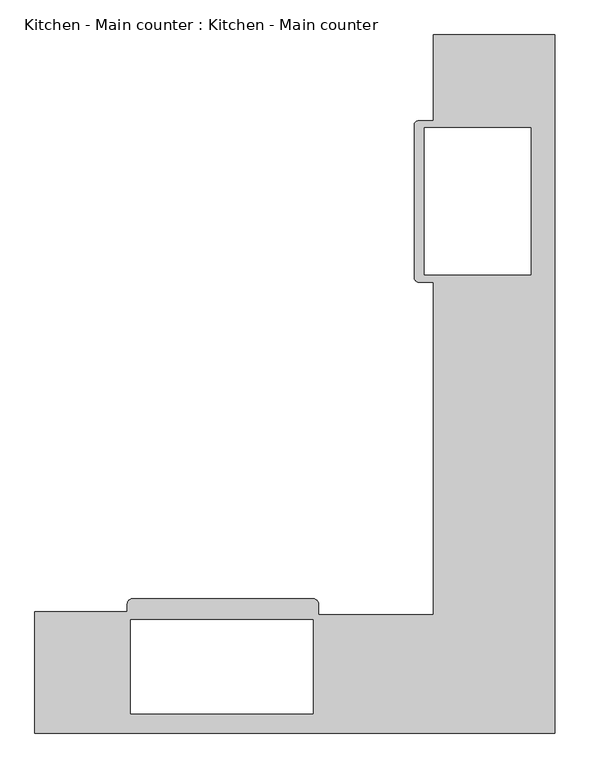
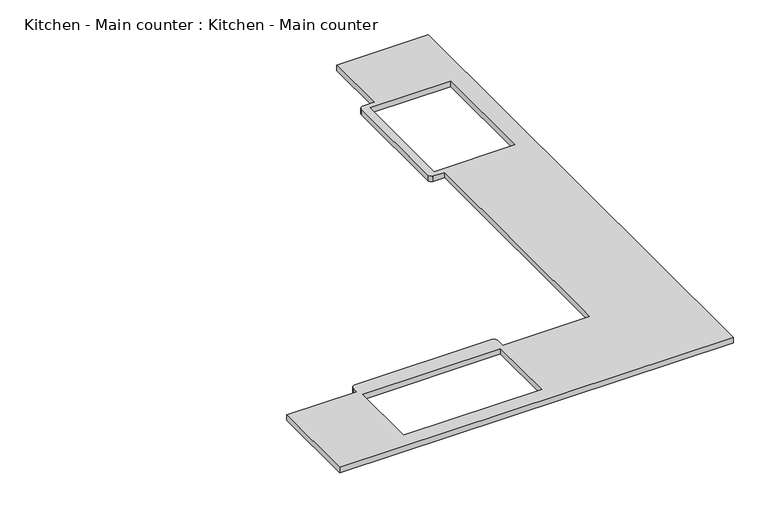
"""IFC4 building model written with IfcOpenShell, lengths in millimetres: furniture geometry, Kitchen - Main counter : Kitchen - Main counter."""

from ifc_helpers import new_model, si_unit, point, frame, frame_2d, origin, place, context, project, spatial, polyline, circle_curve, trimmed, segment, composite_curve, outline, extrude, source, transform, mapped, element, save


def kitchen_main_counter_kitchen_main_counter_9cb608c1(model_context):
    return source(origin(), model_context, "Body", "SweptSolid", [
        extrude(outline(composite_curve([segment(polyline([(5731.3758497, 9294.8125), (6195.1480033, 9294.8125), (6195.1480033, 9332.9125)]), True, "CONTINUOUS"), segment(trimmed(circle_curve(frame_2d((6220.5480033, 9332.9125)), 25.4), [point((6195.1480033, 9332.9125))], [point((6220.5480033, 9358.3125))], False, "CARTESIAN"), True, "CONTINUOUS"), segment(polyline([(6220.5480033, 9358.3125), (7128.4113603, 9358.3125)]), True, "CONTINUOUS"), segment(trimmed(circle_curve(frame_2d((7128.4113603, 9332.9125)), 25.4), [point((7128.4113603, 9358.3125))], [point((7153.8113603, 9332.9125))], False, "CARTESIAN"), True, "CONTINUOUS"), segment(polyline([(7153.8113603, 9332.9125), (7153.8113603, 9278.0953401), (7731.8480033, 9278.0953401), (7731.8480033, 10945.5241338), (7654.0605033, 10945.5241338)]), True, "CONTINUOUS"), segment(trimmed(circle_curve(frame_2d((7661.4688367, 10970.9241338)), 26.4583333), [point((7654.0605033, 10945.5241338))], [point((7635.0105033, 10970.9241338))], False, "CARTESIAN"), True, "CONTINUOUS"), segment(polyline([(7635.0105033, 10970.9241338), (7635.0105033, 11732.9241338)]), True, "CONTINUOUS"), segment(trimmed(circle_curve(frame_2d((7657.4611436, 11732.9241338)), 22.4506403), [point((7635.0105033, 11732.9241338))], [point((7657.4611436, 11755.3747741))], False, "CARTESIAN"), True, "CONTINUOUS"), segment(polyline([(7657.4611436, 11755.3747741), (7731.8480033, 11755.3747741), (7731.8480033, 12185.65), (8339.8605033, 12185.65), (8339.8605033, 8685.2125), (5731.3758497, 8685.2125), (5731.3758497, 9294.8125)]), True, "CONTINUOUS")], self_intersect=False), holes=[polyline([(7685.8105033, 10983.6241338), (8219.2105033, 10983.6241338), (8219.2105033, 11720.2241338), (7685.8105033, 11720.2241338), (7685.8105033, 11351.9241338), (7685.8105033, 10983.6241338)]), polyline([(7126.2875, 9254.5007015), (6211.8875, 9254.5007015), (6211.8875, 8783.3960572), (7126.2875, 8783.3960572), (7126.2875, 9254.5007015)])]), frame((0.0, 0.0, 876.3), z_axis=(0.0, 0.0, 1.0), x_axis=(1.0, 0.0, 0.0)), (0.0, 0.0, 1.0), 38.0405752),
    ])


if __name__ == "__main__":
    model = new_model("IFC4")
    model_context = context("Model", 3, world=origin())
    ifc_project = project(units=[si_unit("LENGTHUNIT", "METRE", prefix="MILLI")], contexts=[model_context])
    site = spatial("IfcSite", under=ifc_project)
    building = spatial("IfcBuilding", under=site)
    placement = place(None, origin())
    kitchen_main_counter_kitchen_main_counter_shape = kitchen_main_counter_kitchen_main_counter_9cb608c1(model_context)
    element("IfcFurniture", 1, ObjectType="Kitchen - Main counter : Kitchen - Main counter", at=placement, inside=building, context=model_context, shape_type="MappedRepresentation", body=[
        mapped(kitchen_main_counter_kitchen_main_counter_shape, transform((0.0, 0.0, 0.0), x_axis=(1.0, 0.0, 0.0), y_axis=(0.0, 1.0, 0.0), z_axis=(0.0, 0.0, 1.0))),
    ])
    save(model, "model.ifc")

# Revit data of these elements
# Type "Kitchen - Main counter : Kitchen - Main counter"
#   COBie.Type = no
# Element 1 (IfcFurniture, "Kitchen - Main counter : Kitchen - Main counter")
#   Materials on its faces: "Corian - Dusk"
# Materials
#   "Corian - Dusk": class "Plastic", colour RGB 75 95 146, transparency 0, Manufacturer = "Corning", Cost = 0
